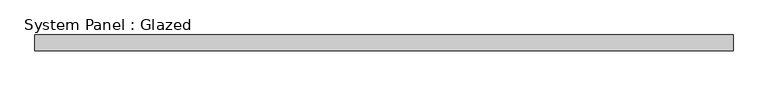
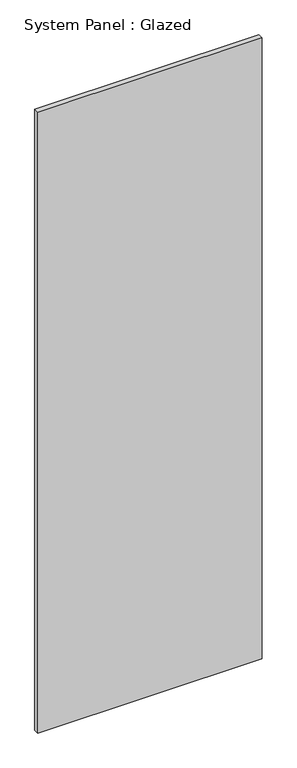
"""IFC4 building model written with IfcOpenShell, lengths in millimetres: plate geometry, System Panel : Glazed."""

from ifc_helpers import new_model, si_unit, origin, origin_with_axes, place, context, project, spatial, polyline, outline, extrude, source, transform, mapped, element, save


def system_panel_glazed_d9a1cec6(model_context):
    return source(origin(), model_context, "Body", "SweptSolid", [
        extrude(outline(polyline([(567.2666667, -44.45), (-567.2666667, -44.45), (-567.2666667, -19.05), (567.2666667, -19.05), (567.2666667, -44.45)])), origin_with_axes(), (0.0, 0.0, 1.0), 3318.9333333),
    ])


if __name__ == "__main__":
    model = new_model("IFC4")
    model_context = context("Model", 3, world=origin())
    ifc_project = project(units=[si_unit("LENGTHUNIT", "METRE", prefix="MILLI")], contexts=[model_context])
    site = spatial("IfcSite", under=ifc_project)
    building = spatial("IfcBuilding", under=site)
    placement = place(None, origin())
    system_panel_glazed_shape = system_panel_glazed_d9a1cec6(model_context)
    element("IfcPlate", 1, ObjectType="System Panel : Glazed", at=placement, inside=building, context=model_context, shape_type="MappedRepresentation", body=[
        mapped(system_panel_glazed_shape, transform((0.0, 0.0, 0.0), x_axis=(1.0, 0.0, 0.0), y_axis=(0.0, 1.0, 0.0), z_axis=(0.0, 0.0, 1.0))),
    ])
    save(model, "model.ifc")

# Revit data of these elements
# Type "System Panel : Glazed"
#   Construction Type Id = "GSP4R"
#   Analytic Construction = "1/8 in Pilkington single glazing"
#   Visual Light Transmittance = 0.9
#   Solar Heat Gain Coefficient = 0.86
#   Heat Transfer Coefficient (U) = 1.18115 BTU/(h·ft²·°F)
#   Define Thermal Properties by = 1
# Element 1 (IfcPlate, "System Panel : Glazed")
#   Materials on its faces: "Glass"
# Materials
#   "Glass": class "Glass", colour RGB 0 128 192, transparency 0.75, Description = "Soda Lime Glass", Cost = 0
